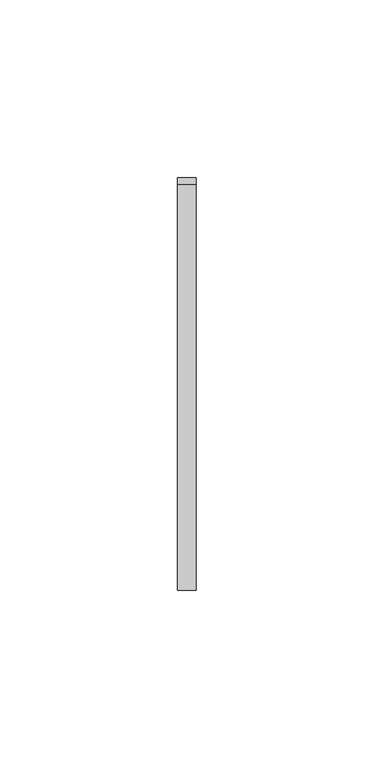
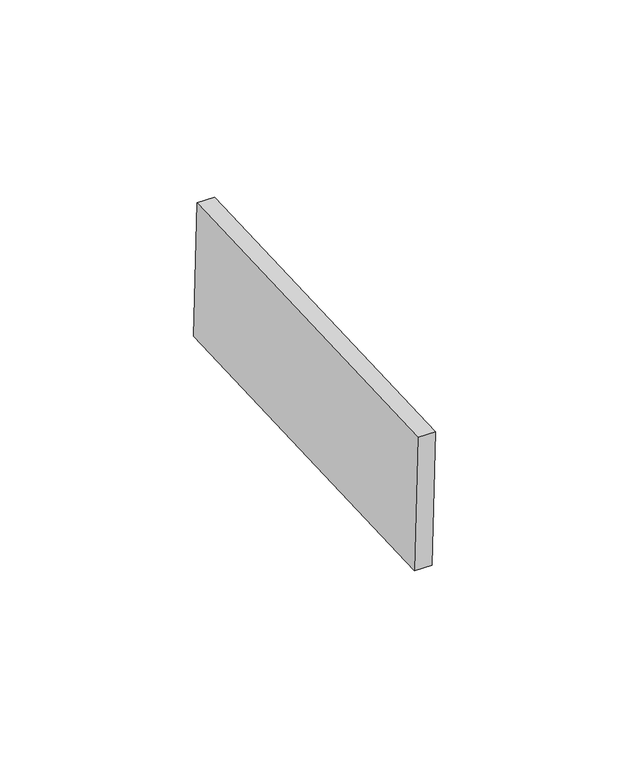
"""IFC4 building model written with IfcOpenShell, lengths in millimetres: proxy geometry, Inner panel:Inner panel:1:Inner panel:1 : Inner panel:Inner panel:300324:2:Inner panel:1:Inner panel:1 : Inner panel:Inner panel:300324:2 : Inner panel:Inner panel:1:Inner panel:1 : Inner panel:Inner panel:300324:300043:99 : Inner panel:Inner panel:1:Inner panel:1 : Inner panel:Inner panel:300324:2:Inner panel:1:Inner panel:1 : Inner panel:Inner panel:300324:2 : Inner panel:Inner panel:1:Inner panel:1 : Inner panel:Inner panel:300324:300043:308120."""

from ifc_helpers import new_model, si_unit, frame, origin, place, context, project, spatial, polyline, outline, extrude, source, transform, mapped, element, save


def generic_models_1a2e485b(model_context):
    return source(origin(), model_context, "Body", "SweptSolid", [
        extrude(outline(polyline([(0.0, -114.3), (0.0, 0.0), (5.2138089, 0.0), (5.2138089, -114.3), (0.0, -114.3)])), frame((592717.395117, -579007.2622385, 3952.103089), z_axis=(0.0, -0.04163054471216399, 0.9991330730923527), x_axis=(-1.0, 0.0, 0.0)), (0.0, 0.0, 1.0), 43.2233908),
    ])


if __name__ == "__main__":
    model = new_model("IFC4")
    model_context = context("Model", 3, world=origin())
    ifc_project = project(units=[si_unit("LENGTHUNIT", "METRE", prefix="MILLI")], contexts=[model_context])
    site = spatial("IfcSite", under=ifc_project)
    building = spatial("IfcBuilding", under=site)
    placement = place(None, origin())
    generic_models_shape = generic_models_1a2e485b(model_context)
    element("IfcBuildingElementProxy", 1, Name="Inner panel:Inner panel:1:Inner panel:1 : Inner panel:Inner panel:300324:2:Inner panel:1:Inner panel:1 : Inner panel:Inner panel:300324:2 : Inner panel:Inner panel:1:Inner panel:1 : Inner panel:Inner panel:300324:300043:99 : Inner panel:Inner panel:1:Inner panel:1 : Inner panel:Inner panel:300324:2:Inner panel:1:Inner panel:1 : Inner panel:Inner panel:300324:2 : Inner panel:Inner panel:1:Inner panel:1 : Inner panel:Inner panel:300324:300043:308120", ObjectType="Inner panel:Inner panel:1:Inner panel:1 : Inner panel:Inner panel:300324:2:Inner panel:1:Inner panel:1 : Inner panel:Inner panel:300324:2 : Inner panel:Inner panel:1:Inner panel:1 : Inner panel:Inner panel:300324:300043:99 : Inner panel:Inner panel:1:Inner panel:1 : Inner panel:Inner panel:300324:2:Inner panel:1:Inner panel:1 : Inner panel:Inner panel:300324:2 : Inner panel:Inner panel:1:Inner panel:1 : Inner panel:Inner panel:300324:300043:308120", at=placement, inside=building, context=model_context, shape_type="MappedRepresentation", body=[
        mapped(generic_models_shape, transform((0.0, 0.0, 0.0), x_axis=(1.0, 0.0, 0.0), y_axis=(0.0, 1.0, 0.0), z_axis=(0.0, 0.0, 1.0))),
    ])
    save(model, "model.ifc")

# Revit data of these elements
# Type "Inner panel:Inner panel:1:Inner panel:1 : Inner panel:Inner panel:300324:2:Inner panel:1:Inner panel:1 : Inner panel:Inner panel:300324:2 : Inner panel:Inner panel:1:Inner panel:1 : Inner panel:Inner panel:300324:300043:99 : Inner panel:Inner panel:1:Inner panel:1 : Inner panel:Inner panel:300324:2:Inner panel:1:Inner panel:1 : Inner panel:Inner panel:300324:2 : Inner panel:Inner panel:1:Inner panel:1 : Inner panel:Inner panel:300324:300043:308120"
#   NameOverride = "Inner panel:Inner panel:1:Inner panel:1 : Inner panel:Inner panel:300324:2:Inner panel:1:Inner panel:1 : Inner panel:Inner panel:300324:2 : Inner panel:Inner panel:1:Inner panel:1 : Inner panel:Inner panel:300324:300043:308120"
#   ObjectTypeOverride = "Inner panel:1:Inner panel:1 : Inner panel:Inner panel:300324:2 : Inner panel:Inner panel:1:Inner panel:1 : Inner panel:Inner panel:300324:300043"
#   Reference = "Inner panel"
#   Tag = "308120"
# Element 1 (IfcBuildingElementProxy, "Inner panel:Inner panel:1:Inner panel:1 : Inner panel:Inner panel:300324:2:Inner panel:1:Inner panel:1 : Inner panel:Inner panel:300324:2 : Inner panel:Inner panel:1:Inner panel:1 : Inner panel:Inner panel:300324:300043:99 : Inner panel:Inner panel:1:Inner panel:1 : Inner panel:Inner panel:300324:2:Inner panel:1:Inner panel:1 : Inner panel:Inner panel:300324:2 : Inner panel:Inner panel:1:Inner panel:1 : Inner panel:Inner panel:300324:300043:308120")
#   Materials on its faces: "SLIDING CLIP"
# Materials
#   "SLIDING CLIP": class "Generic", colour RGB 120 120 120, transparency 0, Cost = 0
